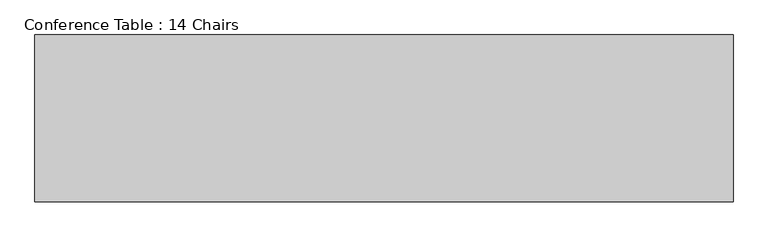
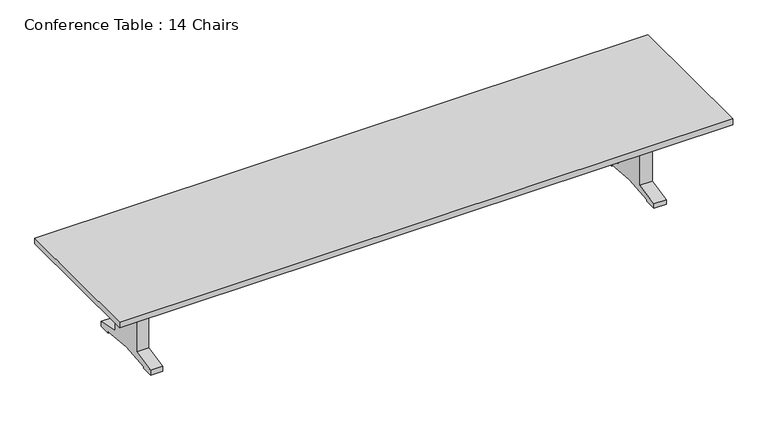
"""IFC4 building model written with IfcOpenShell, lengths in millimetres: furniture geometry, Conference Table : 14 Chairs."""

from ifc_helpers import new_model, si_unit, frame, origin, place, context, project, spatial, polyline, outline, extrude, source, transform, mapped, element, save


def conference_table_14_chairs_0e8207fc(model_context):
    return source(origin(), model_context, "Body", "SweptSolid", [
        extrude(outline(polyline([(-254.0, 0.0), (-355.6, 0.0), (-355.6, 40.4390459), (-152.4, 79.9371247), (-152.4, 555.8555363), (-457.2, 609.6), (-457.2, 711.2), (457.2, 711.2), (457.2, 609.6), (152.4, 555.8555363), (152.4, 79.9371247), (355.6, 40.4390459), (355.6, 0.0), (254.0, 0.0), (254.0, 12.7), (0.0, 34.9221205), (-254.0, 12.7), (-254.0, 0.0)])), frame((2044.7, 0.0, 0.0), z_axis=(1.0, 0.0, 0.0), x_axis=(0.0, 1.0, 0.0)), (0.0, 0.0, 1.0), 101.6),
        extrude(outline(polyline([(-254.0, 0.0), (-355.6, 0.0), (-355.6, 40.4390459), (-152.4, 79.9371247), (-152.4, 555.8555363), (-457.2, 609.6), (-457.2, 711.2), (457.2, 711.2), (457.2, 609.6), (152.4, 555.8555363), (152.4, 79.9371247), (355.6, 40.4390459), (355.6, 0.0), (254.0, 0.0), (254.0, 12.7), (0.0, 34.9221205), (-254.0, 12.7), (-254.0, 0.0)])), frame((-2146.3, 0.0, 0.0), z_axis=(1.0, 0.0, 0.0), x_axis=(0.0, 1.0, 0.0)), (0.0, 0.0, 1.0), 101.6),
        extrude(outline(polyline([(2552.7, -609.6), (-2552.7, -609.6), (-2552.7, 609.6), (2552.7, 609.6), (2552.7, -609.6)])), frame((0.0, 0.0, 711.2), z_axis=(0.0, 0.0, 1.0), x_axis=(1.0, 0.0, 0.0)), (0.0, 0.0, 1.0), 50.8),
        extrude(outline(polyline([(2044.7, 457.2), (2044.7, 419.1), (-2044.7, 419.1), (-2044.7, 457.2), (2044.7, 457.2)])), frame((0.0, 0.0, 609.6), z_axis=(0.0, 0.0, 1.0), x_axis=(1.0, 0.0, 0.0)), (0.0, 0.0, 1.0), 101.6),
        extrude(outline(polyline([(2044.7, -457.2), (-2044.7, -457.2), (-2044.7, -419.1), (2044.7, -419.1), (2044.7, -457.2)])), frame((0.0, 0.0, 609.6), z_axis=(0.0, 0.0, 1.0), x_axis=(1.0, 0.0, 0.0)), (0.0, 0.0, 1.0), 101.6),
    ])


if __name__ == "__main__":
    model = new_model("IFC4")
    model_context = context("Model", 3, world=origin())
    ifc_project = project(units=[si_unit("LENGTHUNIT", "METRE", prefix="MILLI")], contexts=[model_context])
    site = spatial("IfcSite", under=ifc_project)
    building = spatial("IfcBuilding", under=site)
    placement = place(None, origin())
    conference_table_14_chairs_shape = conference_table_14_chairs_0e8207fc(model_context)
    element("IfcFurniture", 1, ObjectType="Conference Table : 14 Chairs", at=placement, inside=building, context=model_context, shape_type="MappedRepresentation", body=[
        mapped(conference_table_14_chairs_shape, transform((0.0, 0.0, 0.0), x_axis=(1.0, 0.0, 0.0), y_axis=(0.0, 1.0, 0.0), z_axis=(0.0, 0.0, 1.0))),
    ])
    save(model, "model.ifc")

# Revit data of these elements
# Type "Conference Table : 14 Chairs"
#   Width = 4' - 0"
#   Length = 16' - 9"
#   Height = 2' - 6"
#   Number of Chairs = 14
#   Number Of Chairs One Side = 6
#   Top = Mahogany
#   Legs and Supports = Mahogany
#   Default Elevation = 0
# Element 1 (IfcFurniture, "Conference Table : 14 Chairs")
#   Materials on its faces: "Mahogany"
# Materials
#   "Mahogany": class "Wood", colour RGB 102 51 32, transparency 0, Description = "Swietenia Macrophylla", Cost = 0
